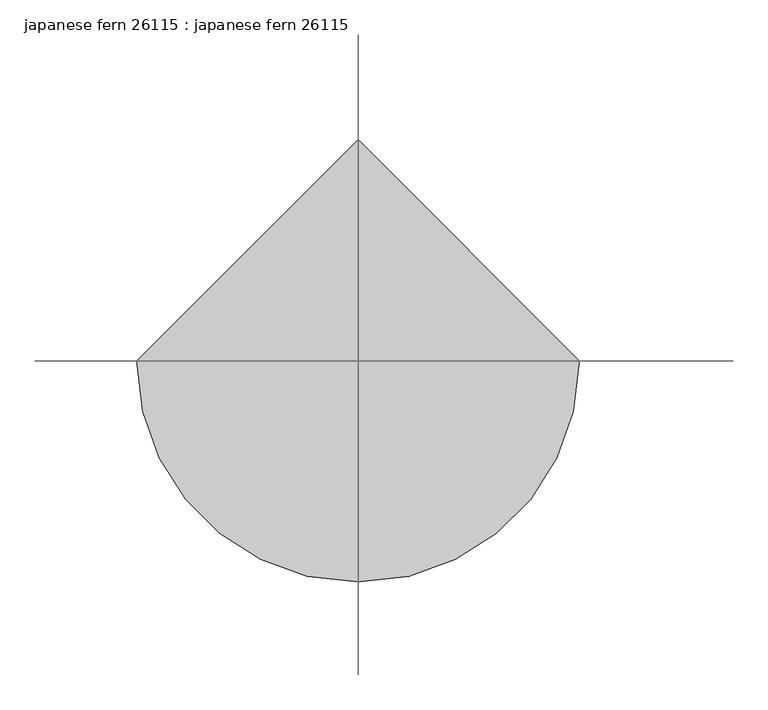
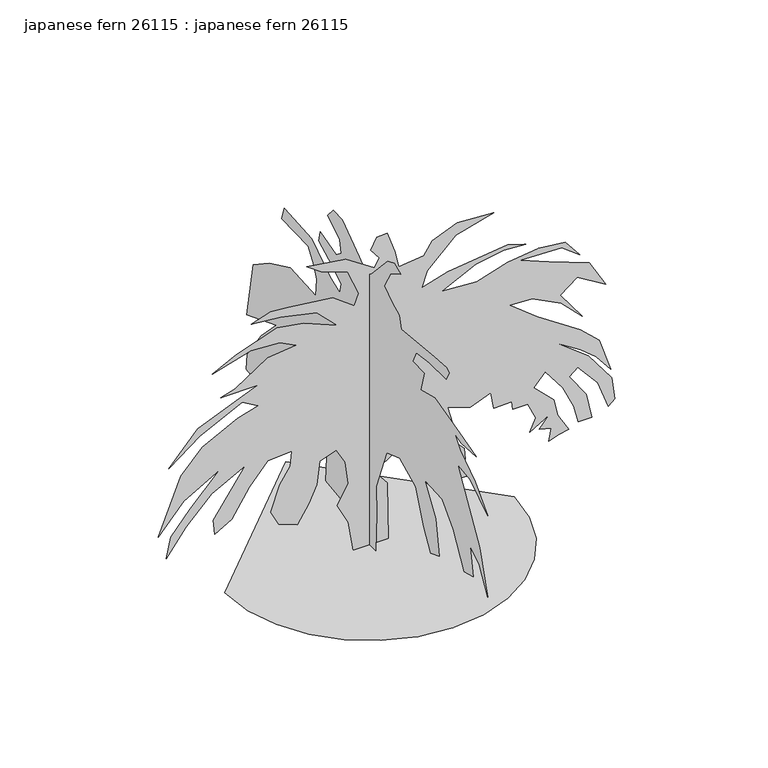
"""IFC4 building model written with IfcOpenShell, lengths in millimetres: proxy geometry, japanese fern 26115 : japanese fern 26115."""

import ifcopenshell
import ifcopenshell.guid

model = None  # the IFC model being written
_history = None  # IfcOwnerHistory: only IFC2X3 demands one
_inside = {}  # id of a spatial element -> (the spatial element, [elements in it])
_under = {}  # id of a project, library or spatial element -> (it, [spatial elements below it])
_declared = {}  # id of a project -> (the project, [libraries it declares])
_typed = {}  # id of a type object -> (the type object, [elements of that type])
_made_of = {}  # id of a material, layer set ... -> (it, [elements and type objects made of it])


def new_model(schema):
    """Start an empty IFC model of exactly this schema.

    Asked for "IFC4X3", IfcOpenShell would pick the latest addendum, in which some entities
    have other attributes; the version numbers below select the first issue.
    IFC2X3 requires an IfcOwnerHistory on every rooted entity: one is made here for all.
    """
    global model, _history
    if schema == "IFC4X3":
        model = ifcopenshell.file(schema_version=(4, 3, 0, 0))
    else:
        model = ifcopenshell.file(schema=schema)
    _inside.clear()
    _under.clear()
    _declared.clear()
    _typed.clear()
    _made_of.clear()
    _history = None
    if model.schema == "IFC2X3":
        org = make("IfcOrganization", Name="unknown")
        user = make(
            "IfcPersonAndOrganization",
            ThePerson=make("IfcPerson", FamilyName="unknown"),
            TheOrganization=org,
        )
        app = make(
            "IfcApplication",
            ApplicationDeveloper=org,
            Version="unknown",
            ApplicationFullName="unknown",
            ApplicationIdentifier="unknown",
        )
        _history = make(
            "IfcOwnerHistory",
            OwningUser=user,
            OwningApplication=app,
            ChangeAction="ADDED",
            CreationDate=0,
        )
    return model


def make(cls, **values):
    """One entity of the class cls with the attributes given. An attribute that is None is left unset."""
    return model.create_entity(
        cls, **{name: value for name, value in values.items() if value is not None}
    )


def rooted(cls, **values):
    """An entity with a GlobalId (a new one), such as an element, a storey or a relation."""
    return make(cls, GlobalId=ifcopenshell.guid.new(), OwnerHistory=_history, **values)


def si_unit(unit_type, name, prefix=None):
    """IfcSIUnit, for example si_unit("LENGTHUNIT", "METRE", prefix="MILLI")."""
    return make("IfcSIUnit", UnitType=unit_type, Prefix=prefix, Name=name)


def assignment(units):
    """IfcUnitAssignment: the units of a project."""
    return None if units is None else make("IfcUnitAssignment", Units=units)


def point(xyz):
    """IfcCartesianPoint."""
    return None if xyz is None else make("IfcCartesianPoint", Coordinates=xyz)


def direction(xyz):
    """IfcDirection."""
    return None if xyz is None else make("IfcDirection", DirectionRatios=xyz)


def frame(location, z_axis=None, x_axis=None):
    """IfcAxis2Placement3D, a coordinate frame: its origin and axes. An axis left out is left unset."""
    return make(
        "IfcAxis2Placement3D",
        Location=point(location),
        Axis=direction(z_axis),
        RefDirection=direction(x_axis),
    )


def origin():
    """The frame at (0, 0, 0) with its axes left unset."""
    return frame((0.0, 0.0, 0.0))


def place(relative_to, where):
    """IfcLocalPlacement: puts the frame where relative to a parent placement (None: the world)."""
    return make(
        "IfcLocalPlacement", PlacementRelTo=relative_to, RelativePlacement=where
    )


def context(
    kind, dimensions, precision=None, world=None, true_north=None, identifier=None
):
    """IfcGeometricRepresentationContext, for example the 3D "Model" context."""
    return make(
        "IfcGeometricRepresentationContext",
        ContextIdentifier=identifier,
        ContextType=kind,
        CoordinateSpaceDimension=dimensions,
        Precision=precision,
        WorldCoordinateSystem=world,
        TrueNorth=true_north,
    )


def project(units=None, contexts=None):
    """IfcProject with its units and contexts."""
    return rooted(
        "IfcProject",
        Name="project",
        RepresentationContexts=contexts,
        UnitsInContext=assignment(units),
    )


def spatial(cls, under=None, at=None, **own):
    """A site, building, storey or space (cls), placed at a placement, below another one or the project."""
    s = rooted(cls, ObjectPlacement=at, **own)
    if under is not None:
        _under.setdefault(under.id(), (under, []))[1].append(s)
    return s


def point_list(points):
    """IfcCartesianPointList2D or 3D."""
    cls = (
        "IfcCartesianPointList2D" if len(points[0]) == 2 else "IfcCartesianPointList3D"
    )
    return make(cls, CoordList=points)


def triangles(points, corners, closed=None, point_numbers=None):
    """IfcTriangulatedFaceSet: each triangle names its three corners, points numbered from 1."""
    return make(
        "IfcTriangulatedFaceSet",
        Coordinates=point_list(points),
        Closed=closed,
        CoordIndex=corners,
        PnIndex=point_numbers,
    )


def shape(context_of_items, identifier, shape_type, items):
    """IfcShapeRepresentation: the items that make up one representation, for example the "Body"."""
    return make(
        "IfcShapeRepresentation",
        ContextOfItems=context_of_items,
        RepresentationIdentifier=identifier,
        RepresentationType=shape_type,
        Items=items,
    )


def source(mapping_origin, context_of_items, identifier, shape_type, items):
    """IfcRepresentationMap: a shape defined once, which mapped items show again and again."""
    return make(
        "IfcRepresentationMap",
        MappingOrigin=mapping_origin,
        MappedRepresentation=shape(context_of_items, identifier, shape_type, items),
    )


def transform(
    local_origin,
    x_axis=None,
    y_axis=None,
    z_axis=None,
    scale=None,
    scale2=None,
    scale3=None,
    uniform=True,
):
    """IfcCartesianTransformationOperator3D, or its non-uniform kind. x_axis, y_axis, z_axis: its Axis1, 2, 3."""
    if uniform:
        return make(
            "IfcCartesianTransformationOperator3D",
            Axis1=direction(x_axis),
            Axis2=direction(y_axis),
            LocalOrigin=point(local_origin),
            Scale=scale,
            Axis3=direction(z_axis),
        )
    return make(
        "IfcCartesianTransformationOperator3DnonUniform",
        Axis1=direction(x_axis),
        Axis2=direction(y_axis),
        LocalOrigin=point(local_origin),
        Scale=scale,
        Axis3=direction(z_axis),
        Scale2=scale2,
        Scale3=scale3,
    )


def mapped(mapping_source, mapping_target):
    """IfcMappedItem: shows the shape of a source again, moved by a transform."""
    return make(
        "IfcMappedItem", MappingSource=mapping_source, MappingTarget=mapping_target
    )


def made_of(thing, what):
    """Note that an element or type object is made of a material, layer set ...; save() writes the relation."""
    if what is not None:
        _made_of.setdefault(what.id(), (what, []))[1].append(thing)
    return thing


def element(
    cls,
    number,
    at=None,
    inside=None,
    cuts=None,
    type_object=None,
    material=None,
    context=None,
    identifier="Body",
    shape_type=None,
    held_by="IfcProductDefinitionShape",
    body=None,
    shapes=None,
    **own,
):
    """One element of the class cls, such as IfcWall. Its Tag is "e" and its number.

    at: its placement. inside: the storey or other place that contains it. cuts: it is an
    opening in that element (IfcRelVoidsElement). A single representation is given by context,
    identifier, shape_type and body (its items); several are given by shapes. held_by: the class
    of the entity that holds the representations. save() writes the other relations.
    """
    e = rooted(cls, Tag="e%d" % number, ObjectPlacement=at, **own)
    if body is not None:
        shapes = [shape(context, identifier, shape_type, body)]
    if shapes is not None:
        e.Representation = make(held_by, Representations=shapes)
    if inside is not None:
        _inside.setdefault(inside.id(), (inside, []))[1].append(e)
    if cuts is not None:
        rooted(
            "IfcRelVoidsElement", RelatingBuildingElement=cuts, RelatedOpeningElement=e
        )
    if type_object is not None:
        _typed.setdefault(type_object.id(), (type_object, []))[1].append(e)
    return made_of(e, material)


def aggregate(whole, parts):
    """IfcRelAggregates: a whole, such as a stair, and the parts it consists of."""
    return rooted("IfcRelAggregates", RelatingObject=whole, RelatedObjects=parts)


def save(model, path):
    """Write the relations noted so far, then the file.

    IfcRelAggregates (storeys below a building ...), IfcRelContainedInSpatialStructure (elements
    in a storey), IfcRelDefinesByType, IfcRelAssociatesMaterial and IfcRelDeclares: one each for
    every whole, place, type object, material and project.
    """
    for whole, parts in _under.values():
        aggregate(whole, parts)
    for where, things in _inside.values():
        rooted(
            "IfcRelContainedInSpatialStructure",
            RelatedElements=things,
            RelatingStructure=where,
        )
    for kind, things in _typed.values():
        rooted("IfcRelDefinesByType", RelatedObjects=things, RelatingType=kind)
    for what, things in _made_of.values():
        rooted("IfcRelAssociatesMaterial", RelatedObjects=things, RelatingMaterial=what)
    for by, libraries in _declared.values():
        rooted("IfcRelDeclares", RelatingContext=by, RelatedDefinitions=libraries)
    model.write(path)


def japanese_fern_26115_japanese_fern_26115_30b4c15b(model_context):
    return source(origin(), model_context, "Body", "Tessellation", [
        triangles([(-340.212337, 0.0, 2.34e-05), (-331.2181912, -77.9542988, 2.34e-05), (-305.6048564, -149.5428615, 2.34e-05), (-265.4195731, -212.7146324, 2.34e-05), (-212.7146324, -265.4195731, 2.34e-05), (-149.5428615, -305.6048564, 2.34e-05), (-77.9542988, -331.2181912, 2.34e-05), (1.49e-05, -340.212337, 2.34e-05), (77.9542988, -331.2181912, 2.34e-05), (149.5428615, -305.6048564, 2.34e-05), (212.7146324, -265.4195731, 2.34e-05), (265.4195731, -212.7146324, 2.34e-05), (305.6048564, -149.5428615, 2.34e-05), (331.2181912, -77.9542988, 2.34e-05), (340.212337, 2.97e-05, 2.34e-05), (-4.46e-05, 340.212337, 2.34e-05), (-37.8980319, 2.29e-05, 3.6e-06), (-50.0874814, 2.41e-05, 73.5418183), (-75.8826774, 2.22e-05, 123.7339445), (-49.5540792, 1.83e-05, 170.5209506), (-56.979003, 1.53e-05, 225.9335385), (-77.3492758, 1.4e-05, 262.2445852), (-116.2627981, 1.66e-05, 248.3474865), (-123.5028085, 2.02e-05, 192.7652324), (-143.0648503, 2.35e-05, 151.8270789), (-169.0734009, 2.72e-05, 109.3715308), (-213.7047246, 2.81e-05, 126.2541304), (-232.5443813, 2.67e-05, 163.0480237), (-210.7659323, 2.22e-05, 223.3318078), (-185.9735321, 1.89e-05, 260.6164324), (-182.3167059, 1.66e-05, 296.5396212), (-238.5613832, 1.93e-05, 292.8185184), (-282.7321973, 2.42e-05, 242.1521888), (-323.5728004, 2.99e-05, 177.126216), (-363.5396922, 3.3e-05, 153.4968807), (-367.1566226, 3.1e-05, 190.2732333), (-291.3732759, 2.12e-05, 298.3785896), (-370.9310652, 2.72e-05, 256.7835813), (-430.3492407, 3.34e-05, 195.5366293), (-477.8725754, 3.92e-05, 133.2528402), (-467.4636904, 3.58e-05, 182.8625483), (-420.8344145, 3.05e-05, 237.2243282), (-351.5280344, 2.32e-05, 310.1438599), (-436.732245, 2.98e-05, 261.3606638), (-497.0571965, 3.65e-05, 192.7571115), (-443.5089389, 2.62e-05, 326.4709519), (-392.9096655, 2.08e-05, 380.0648827), (-309.8949288, 1.46e-05, 423.094996), (-260.7967811, 1.16e-05, 437.3545544), (-299.3412489, 1.2e-05, 459.500768), (-398.9192914, 1.93e-05, 409.5872812), (-471.8705798, 2.58e-05, 354.6903414), (-403.1941031, 1.83e-05, 430.1180775), (-300.6061608, 1.12e-05, 473.1100754), (-262.5823916, 8.7e-06, 488.4237482), (-349.0058046, 1.24e-05, 488.2357873), (-315.6607106, 1.04e-05, 498.3805169), (-238.5613832, 4e-06, 548.5353044), (-172.4069002, 6e-07, 556.9452561), (-210.7659323, 1.1e-06, 576.3305191), (-278.7875798, 3.9e-06, 580.4732532), (-369.1987945, 9.4e-06, 554.0953574), (-313.0699167, 5.2e-06, 582.9446503), (-216.6861742, -1e-06, 616.0738781), (-154.0988607, -3.1e-06, 605.5227053), (-75.0741966, -4.5e-06, 572.1420393), (-123.4916265, -5.3e-06, 620.6382071), (-209.0953766, -2.7e-06, 638.8728498), (-277.4743968, -1e-07, 645.8171934), (-232.2393309, -3e-06, 661.5423237), (-190.0088236, -4.6e-06, 657.7145777), (-85.7208487, -8.4e-06, 644.6056395), (-35.6564855, -8.3e-06, 606.9044523), (-24.5384073, -1.05e-05, 634.6996307), (-50.8667489, -1.3e-05, 696.1980572), (-113.4009815, -1.16e-05, 718.2401711), (-146.8372491, -1.16e-05, 743.1016623), (-55.5814956, -1.48e-05, 730.2366045), (11.5952668, -1.5e-05, 684.7325506), (23.1518731, -1.68e-05, 706.0913486), (3.2567592, -1.75e-05, 731.9840996), (17.6289544, -1.97e-05, 758.3441912), (41.4979712, -2.09e-05, 760.5615704), (59.6452374, -1.86e-05, 708.9971306), (68.5156716, -1.65e-05, 668.0955574), (127.4710438, -1.95e-05, 674.2321741), (147.7915331, -2.21e-05, 704.1889212), (206.1616894, -2.62e-05, 729.2028013), (292.3257614, -2.96e-05, 723.6452917), (202.8348031, -2.42e-05, 698.6847513), (136.1791696, -1.75e-05, 634.3440565), (123.7575623, -1.46e-05, 595.466851), (183.9252741, -1.84e-05, 615.2432602), (325.6810292, -2.56e-05, 631.9208759), (367.486835, -2.67e-05, 619.3809437), (315.6911957, -2.46e-05, 622.1876038), (249.7079049, -2.1e-05, 609.8203354), (170.7500609, -1.52e-05, 570.6967787), (252.258585, -1.85e-05, 566.1527246), (325.6530876, -2.3e-05, 588.2608592), (397.9490381, -2.68e-05, 598.5656445), (460.1815041, -2.91e-05, 591.0853598), (495.2309272, -2.81e-05, 548.5353044), (452.9501141, -2.81e-05, 580.5189626), (355.0433722, -2.4e-05, 583.2977174), (420.1841635, -2.53e-05, 556.8741122), (516.8336057, -2.73e-05, 520.4505724), (556.2848313, -2.51e-05, 453.460657), (489.3051261, -2.46e-05, 494.41557), (449.4220591, -2.1e-05, 463.6816175), (500.7909802, -1.9e-05, 392.8817239), (450.7580967, -1.98e-05, 442.9146074), (383.0951119, -1.89e-05, 477.7430411), (329.99392, -1.68e-05, 480.9358332), (395.1677399, -1.66e-05, 429.0157465), (495.6652757, -1.69e-05, 361.8734422), (541.06265, -1.64e-05, 319.2167072), (567.5802175, -1.27e-05, 237.3833302), (533.9328526, -1.38e-05, 280.9008592), (497.6007317, -1.4e-05, 310.7127932), (440.194243, -1.36e-05, 346.6664852), (514.6872977, -1.35e-05, 290.0397636), (570.595186, -1.15e-05, 215.9856355), (576.6531012, -8.5e-06, 161.5684811), (561.938883, -7.1e-06, 148.2847988), (536.9249665, -1e-05, 214.9932542), (489.6734176, -1.12e-05, 270.583393), (469.5464848, -9.4e-06, 254.0962635), (510.5775922, -7.7e-06, 195.5264555), (523.0261056, -4.6e-06, 134.3872005), (491.7079591, -3.2e-06, 133.6020922), (481.1339315, -5.3e-06, 176.3159639), (454.7662096, -7.4e-06, 231.6510674), (413.5344604, -8.8e-06, 285.1248746), (386.501263, -5.8e-06, 255.5745526), (434.0830244, -5.2e-06, 209.4342185), (443.1813063, -3e-06, 166.6068182), (468.6523896, -1.6e-06, 123.9640722), (446.3842358, -3e-07, 118.289464), (421.5049404, 1.3e-06, 110.591996), (428.004798, -8e-07, 139.9015351), (399.5416008, 0.0, 147.6790127), (422.9629183, -2.7e-06, 176.0799863), (377.2150203, 9e-07, 148.592647), (391.2256476, -1.5e-06, 179.1531272), (372.9656067, -3.1e-06, 218.8891102), (336.6588839, -1.5e-06, 219.0854463), (334.8783603, -2.6e-06, 238.301043), (292.3257614, -6e-07, 237.2294151), (285.8309907, -2.8e-06, 277.7512695), (236.7361495, 5e-07, 259.4658122), (183.9252741, 1.8e-06, 276.1434461), (200.6023993, 4.7e-06, 214.9932542), (199.418242, 6.4e-06, 187.1818159), (222.8385421, 6.9e-06, 162.1823971), (225.6180599, 8.4e-06, 134.3872005), (208.5548754, 9.9e-06, 121.5754553), (237.8440942, 1.05e-05, 90.4480402), (182.0385615, 1.28e-05, 92.8412262), (191.5158174, 1e-05, 133.3458033), (165.4579784, 1e-05, 152.2179799), (173.5882597, 8.2e-06, 176.3515177), (109.0494575, 1.14e-05, 169.6062899), (94.9809212, 1.06e-05, 192.7571115), (145.0122605, 6.8e-06, 220.5522899), (83.3228392, 9.3e-06, 223.7369429), (11.6764698, 1.52e-05, 177.2189248), (42.170055, 1.61e-05, 139.9462362), (44.9495728, 1.82e-05, 0.0), (0.00212, 26.6938489, 3.6e-06), (0.0021253, 22.2078332, 125.235588), (0.0021271, 60.1697466, 128.8281648), (0.002126, 119.4035039, 42.9622804), (0.0021289, 177.9956579, 51.1230378), (0.0021314, 173.4581986, 113.1355544), (0.0021337, 137.5657583, 202.421547), (0.0021299, 136.57414, 252.5593115), (0.0021317, 167.407932, 262.8744886), (0.0021371, 226.3958104, 190.2732333), (0.0021373, 288.3557457, 133.4656906), (0.0021388, 315.632769, 140.3605096), (0.0021407, 309.8923854, 190.0641981), (0.0021433, 346.6360002, 212.5124464), (0.0021443, 409.4094941, 172.1231784), (0.0021442, 453.2701527, 125.235588), (0.0021466, 501.6723581, 132.7981805), (0.0021481, 497.133391, 172.1231784), (0.0021432, 441.1721629, 252.2857635), (0.0021433, 378.8939512, 316.9053294), (0.0021465, 498.6472157, 270.4360728), (0.0021515, 472.2337844, 410.5144049), (0.0021506, 407.8956694, 453.4479761), (0.0021486, 323.1969149, 492.7747544), (0.0021437, 217.6417118, 487.9487409), (0.0021455, 214.2957677, 530.5851645), (0.0021473, 226.9167634, 559.1017015), (0.0021497, 249.3380874, 591.8626016), (0.0021545, 357.9821463, 594.1105021), (0.0021554, 347.3954378, 625.8731346), (0.0021502, 235.3830889, 618.7560545), (0.0021449, 161.3091401, 570.0389337), (0.0021424, 119.7014417, 554.0699593), (0.0021433, 115.4461873, 579.5537599), (0.0021468, 165.8956152, 609.2361777), (0.0021495, 206.7331843, 630.4121017), (0.0021444, 199.1706008, 657.6358034), (0.0021408, 134.2553771, 640.0184195), (0.0021406, 114.4705746, 656.1245584), (0.0021422, 120.4276329, 685.149095), (0.0021457, 170.4330744, 716.6247173), (0.0021458, 147.7455603, 742.3371014), (0.0021442, 111.4454322, 740.823313), (0.002139, 41.6899925, 691.1155186), (0.0021365, 10.7464246, 665.9695244), (0.0021362, -10.1176737, 680.5009048), (0.0021365, -74.5923583, 749.8987038), (0.0021358, -101.8173226, 761.9992733), (0.0021341, -127.5299701, 749.8987038), (0.0021349, -87.1447716, 726.4240465), (0.002134, -60.7928054, 680.9606152), (0.0021316, -92.5270285, 657.5951809), (0.0021298, -121.8045655, 644.2526087), (0.0021341, -129.7537351, 615.210268), (0.0021228, -265.1681168, 628.8983133), (0.0021208, -315.0816035, 631.9234194), (0.00212, -325.668312, 624.3618896), (0.0021255, -313.5677788, 601.6746117), (0.0021285, -243.6485001, 600.9557965), (0.0021305, -191.8444855, 593.8259992), (0.0021298, -176.5968879, 563.282551), (0.0021277, -223.3409642, 562.4341653), (0.0021262, -209.0156213, 512.3124063), (0.0021243, -266.6794162, 527.5625656), (0.0021188, -366.5470304, 501.9288832), (0.002115, -434.5681692, 482.1855025), (0.0021175, -375.2998755, 480.0595058), (0.002119, -348.4190672, 487.3848581), (0.0021168, -370.0115719, 459.7014462), (0.0021124, -430.801357, 418.7795254), (0.0021078, -482.9678312, 365.7240792), (0.0021129, -410.4102324, 411.3017841), (0.0021154, -360.3773852, 417.8549815), (0.0021108, -398.4519507, 351.1901917), (0.0021049, -449.6938448, 265.8970875), (0.0021049, -481.8349789, 162.1823971), (0.002103, -448.18002, 222.0356478), (0.0021056, -410.473746, 244.4529204), (0.0021022, -423.4226649, 177.6834858), (0.0021093, -387.3318446, 167.7414328), (0.0021087, -342.3053052, 246.2357331), (0.0021128, -296.4634267, 293.7202257), (0.0021161, -226.1207364, 298.3785896), (0.0021111, -271.2183834, 229.5982494), (0.0021128, -284.3374772, 144.5642138), (0.0021137, -249.3695898, 130.0336417), (0.002117, -221.7963819, 179.3619262), (0.002116, -188.1828268, 259.1153067), (0.0021202, -123.9887073, 290.1007337), (0.0021217, -70.0716722, 271.1447323), (0.0021248, -27.498267, 162.3606929), (0.0021217, -30.4360283, 94.6027103), (0.0021177, -25.7012178, 2.43e-05)], [[15, 16, 1], [14, 15, 1], [14, 1, 2], [13, 14, 2], [13, 2, 3], [13, 3, 4], [12, 13, 4], [11, 12, 4], [11, 4, 5], [11, 5, 6], [11, 6, 7], [11, 7, 8], [11, 8, 9], [11, 9, 10], [110, 111, 112], [51, 52, 53], [61, 62, 63], [102, 103, 104], [94, 95, 96], [55, 56, 57], [88, 89, 90], [44, 45, 46], [117, 118, 119], [61, 63, 64], [68, 69, 70], [39, 40, 41], [107, 108, 109], [76, 77, 78], [39, 41, 42], [75, 76, 78], [38, 39, 42], [38, 42, 43], [60, 61, 64], [143, 144, 145], [93, 94, 96], [93, 96, 97], [93, 97, 98], [68, 70, 71], [37, 38, 43], [55, 57, 58], [157, 158, 159], [157, 159, 160], [75, 78, 79], [92, 93, 98], [74, 75, 79], [67, 68, 71], [67, 71, 72], [110, 112, 113], [139, 140, 141], [87, 88, 90], [87, 90, 91], [86, 87, 91], [117, 119, 120], [116, 117, 120], [116, 120, 121], [115, 116, 121], [101, 102, 104], [101, 104, 105], [100, 101, 105], [106, 107, 109], [34, 35, 36], [141, 142, 143], [43, 44, 46], [43, 46, 47], [124, 125, 126], [123, 124, 126], [122, 123, 126], [122, 126, 127], [34, 36, 37], [33, 34, 37], [32, 33, 37], [60, 64, 65], [59, 60, 65], [137, 138, 139], [137, 139, 141], [137, 141, 143], [136, 137, 143], [121, 122, 127], [50, 51, 53], [50, 53, 54], [66, 67, 72], [66, 72, 73], [106, 109, 110], [106, 110, 113], [129, 130, 131], [129, 131, 132], [129, 132, 133], [128, 129, 133], [128, 133, 134], [43, 47, 48], [37, 43, 48], [105, 106, 113], [105, 113, 114], [100, 105, 114], [99, 100, 114], [59, 65, 66], [163, 164, 165], [162, 163, 165], [168, 169, 17], [168, 17, 18], [168, 18, 19], [168, 19, 20], [167, 168, 20], [167, 20, 21], [146, 147, 148], [121, 127, 128], [121, 128, 134], [85, 86, 91], [148, 149, 150], [37, 48, 49], [32, 37, 49], [31, 32, 49], [85, 91, 92], [25, 26, 27], [25, 27, 28], [25, 28, 29], [24, 25, 29], [24, 29, 30], [23, 24, 30], [23, 30, 31], [136, 143, 145], [135, 136, 145], [135, 145, 146], [135, 146, 148], [82, 83, 84], [81, 82, 84], [80, 81, 84], [80, 84, 85], [79, 80, 85], [50, 54, 55], [49, 50, 55], [160, 161, 162], [156, 157, 160], [155, 156, 160], [155, 160, 162], [154, 155, 162], [154, 162, 165], [153, 154, 165], [152, 153, 165], [74, 79, 85], [74, 85, 92], [73, 74, 92], [166, 167, 21], [55, 58, 59], [166, 21, 22], [152, 165, 166], [135, 148, 150], [134, 135, 150], [121, 134, 150], [115, 121, 150], [114, 115, 150], [114, 150, 151], [114, 151, 152], [99, 114, 152], [98, 99, 152], [98, 152, 166], [98, 166, 22], [92, 98, 22], [73, 92, 22], [66, 73, 22], [59, 66, 22], [55, 59, 22], [49, 55, 22], [31, 49, 22], [23, 31, 22], [244, 245, 246], [239, 240, 241], [234, 235, 236], [234, 236, 237], [233, 234, 237], [238, 239, 241], [238, 241, 242], [217, 218, 219], [216, 217, 219], [189, 190, 191], [244, 246, 247], [215, 216, 219], [215, 219, 220], [197, 198, 199], [197, 199, 200], [230, 231, 232], [189, 191, 192], [209, 210, 211], [209, 211, 212], [209, 212, 213], [208, 209, 213], [197, 200, 201], [196, 197, 201], [195, 196, 201], [243, 244, 247], [262, 170, 171], [261, 262, 171], [260, 261, 171], [205, 206, 207], [204, 205, 207], [203, 204, 207], [185, 186, 187], [184, 185, 187], [184, 187, 188], [183, 184, 188], [183, 188, 189], [173, 174, 175], [172, 173, 175], [172, 175, 176], [247, 248, 249], [247, 249, 250], [243, 247, 250], [243, 250, 251], [242, 243, 251], [254, 255, 256], [253, 254, 256], [253, 256, 257], [252, 253, 257], [225, 226, 227], [224, 225, 227], [224, 227, 228], [223, 224, 228], [223, 228, 229], [223, 229, 230], [180, 181, 182], [179, 180, 182], [189, 192, 193], [189, 193, 194], [252, 257, 258], [203, 207, 208], [242, 251, 252], [208, 213, 214], [203, 208, 214], [183, 189, 194], [182, 183, 194], [179, 182, 194], [178, 179, 194], [177, 178, 194], [195, 201, 202], [194, 195, 202], [177, 194, 202], [237, 238, 242], [237, 242, 252], [233, 237, 252], [232, 233, 252], [232, 252, 258], [230, 232, 258], [230, 258, 259], [223, 230, 259], [221, 222, 223], [221, 223, 259], [220, 221, 259], [215, 220, 259], [214, 215, 259], [203, 214, 259], [202, 203, 259], [177, 202, 259], [177, 259, 260], [176, 177, 260], [172, 176, 260], [172, 260, 171]], closed=False),
    ])


if __name__ == "__main__":
    model = new_model("IFC4")
    model_context = context("Model", 3, world=origin())
    ifc_project = project(units=[si_unit("LENGTHUNIT", "METRE", prefix="MILLI")], contexts=[model_context])
    site = spatial("IfcSite", under=ifc_project)
    building = spatial("IfcBuilding", under=site)
    placement = place(None, origin())
    japanese_fern_26115_japanese_fern_26115_shape = japanese_fern_26115_japanese_fern_26115_30b4c15b(model_context)
    element("IfcBuildingElementProxy", 1, Name="japanese fern 26115 : japanese fern 26115", ObjectType="japanese fern 26115 : japanese fern 26115", at=placement, inside=building, context=model_context, shape_type="MappedRepresentation", body=[
        mapped(japanese_fern_26115_japanese_fern_26115_shape, transform((0.0, 0.0, 0.0), x_axis=(1.0, 0.0, 0.0), y_axis=(0.0, 1.0, 0.0), z_axis=(0.0, 0.0, 1.0))),
    ])
    save(model, "model.ifc")

# Revit data of these elements
# Type "japanese fern 26115 : japanese fern 26115"
#   built-in parameter 1005195 = "RPC-16-G1GK-JAPX-7J4P-Q000-ST1L-LVER-AU"
#   Height = 0
